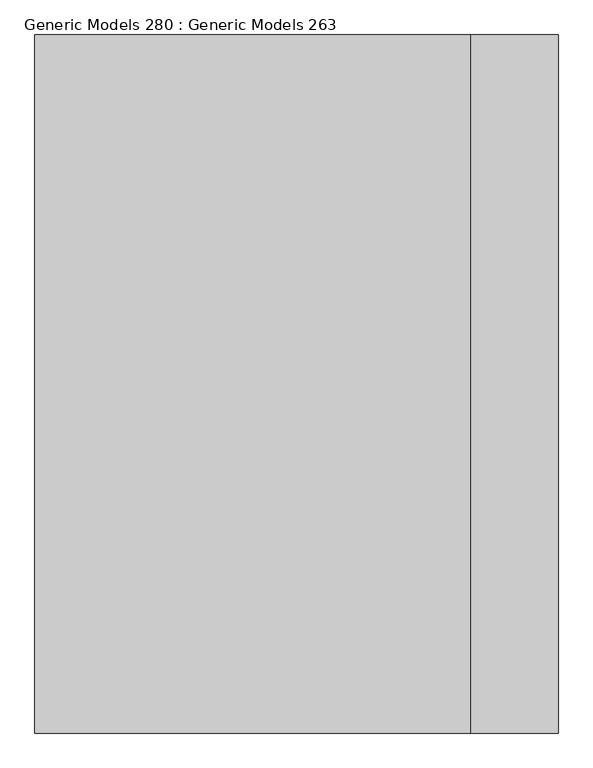
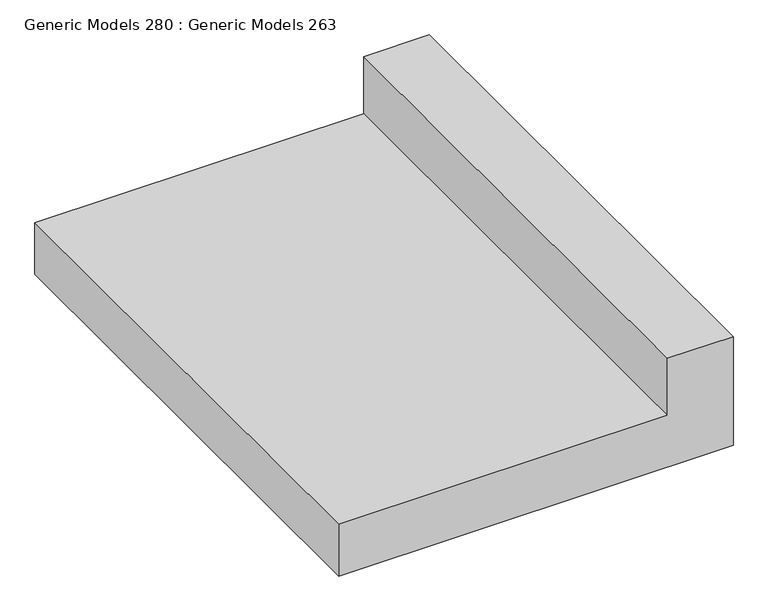
"""IFC4 building model written with IfcOpenShell, lengths in millimetres: proxy geometry, Generic Models 280 : Generic Models 263."""

import ifcopenshell
import ifcopenshell.guid

model = None  # the IFC model being written
_history = None  # IfcOwnerHistory: only IFC2X3 demands one
_inside = {}  # id of a spatial element -> (the spatial element, [elements in it])
_under = {}  # id of a project, library or spatial element -> (it, [spatial elements below it])
_declared = {}  # id of a project -> (the project, [libraries it declares])
_typed = {}  # id of a type object -> (the type object, [elements of that type])
_made_of = {}  # id of a material, layer set ... -> (it, [elements and type objects made of it])


def new_model(schema):
    """Start an empty IFC model of exactly this schema.

    Asked for "IFC4X3", IfcOpenShell would pick the latest addendum, in which some entities
    have other attributes; the version numbers below select the first issue.
    IFC2X3 requires an IfcOwnerHistory on every rooted entity: one is made here for all.
    """
    global model, _history
    if schema == "IFC4X3":
        model = ifcopenshell.file(schema_version=(4, 3, 0, 0))
    else:
        model = ifcopenshell.file(schema=schema)
    _inside.clear()
    _under.clear()
    _declared.clear()
    _typed.clear()
    _made_of.clear()
    _history = None
    if model.schema == "IFC2X3":
        org = make("IfcOrganization", Name="unknown")
        user = make(
            "IfcPersonAndOrganization",
            ThePerson=make("IfcPerson", FamilyName="unknown"),
            TheOrganization=org,
        )
        app = make(
            "IfcApplication",
            ApplicationDeveloper=org,
            Version="unknown",
            ApplicationFullName="unknown",
            ApplicationIdentifier="unknown",
        )
        _history = make(
            "IfcOwnerHistory",
            OwningUser=user,
            OwningApplication=app,
            ChangeAction="ADDED",
            CreationDate=0,
        )
    return model


def make(cls, **values):
    """One entity of the class cls with the attributes given. An attribute that is None is left unset."""
    return model.create_entity(
        cls, **{name: value for name, value in values.items() if value is not None}
    )


def rooted(cls, **values):
    """An entity with a GlobalId (a new one), such as an element, a storey or a relation."""
    return make(cls, GlobalId=ifcopenshell.guid.new(), OwnerHistory=_history, **values)


def si_unit(unit_type, name, prefix=None):
    """IfcSIUnit, for example si_unit("LENGTHUNIT", "METRE", prefix="MILLI")."""
    return make("IfcSIUnit", UnitType=unit_type, Prefix=prefix, Name=name)


def assignment(units):
    """IfcUnitAssignment: the units of a project."""
    return None if units is None else make("IfcUnitAssignment", Units=units)


def point(xyz):
    """IfcCartesianPoint."""
    return None if xyz is None else make("IfcCartesianPoint", Coordinates=xyz)


def direction(xyz):
    """IfcDirection."""
    return None if xyz is None else make("IfcDirection", DirectionRatios=xyz)


def frame(location, z_axis=None, x_axis=None):
    """IfcAxis2Placement3D, a coordinate frame: its origin and axes. An axis left out is left unset."""
    return make(
        "IfcAxis2Placement3D",
        Location=point(location),
        Axis=direction(z_axis),
        RefDirection=direction(x_axis),
    )


def origin():
    """The frame at (0, 0, 0) with its axes left unset."""
    return frame((0.0, 0.0, 0.0))


def place(relative_to, where):
    """IfcLocalPlacement: puts the frame where relative to a parent placement (None: the world)."""
    return make(
        "IfcLocalPlacement", PlacementRelTo=relative_to, RelativePlacement=where
    )


def context(
    kind, dimensions, precision=None, world=None, true_north=None, identifier=None
):
    """IfcGeometricRepresentationContext, for example the 3D "Model" context."""
    return make(
        "IfcGeometricRepresentationContext",
        ContextIdentifier=identifier,
        ContextType=kind,
        CoordinateSpaceDimension=dimensions,
        Precision=precision,
        WorldCoordinateSystem=world,
        TrueNorth=true_north,
    )


def project(units=None, contexts=None):
    """IfcProject with its units and contexts."""
    return rooted(
        "IfcProject",
        Name="project",
        RepresentationContexts=contexts,
        UnitsInContext=assignment(units),
    )


def spatial(cls, under=None, at=None, **own):
    """A site, building, storey or space (cls), placed at a placement, below another one or the project."""
    s = rooted(cls, ObjectPlacement=at, **own)
    if under is not None:
        _under.setdefault(under.id(), (under, []))[1].append(s)
    return s


def polyline(points):
    """IfcPolyline through the points."""
    return make("IfcPolyline", Points=[point(p) for p in points])


def outline(outer, holes=None, kind="AREA"):
    """IfcArbitraryClosedProfileDef: a profile drawn as a closed curve; with holes, ...WithVoids."""
    if holes is None:
        return make("IfcArbitraryClosedProfileDef", ProfileType=kind, OuterCurve=outer)
    return make(
        "IfcArbitraryProfileDefWithVoids",
        ProfileType=kind,
        OuterCurve=outer,
        InnerCurves=holes,
    )


def extrude(swept, where, along, depth):
    """IfcExtrudedAreaSolid: the profile swept, set in the frame where, extruded along a direction by depth."""
    return make(
        "IfcExtrudedAreaSolid",
        SweptArea=swept,
        Position=where,
        ExtrudedDirection=direction(along),
        Depth=depth,
    )


def shape(context_of_items, identifier, shape_type, items):
    """IfcShapeRepresentation: the items that make up one representation, for example the "Body"."""
    return make(
        "IfcShapeRepresentation",
        ContextOfItems=context_of_items,
        RepresentationIdentifier=identifier,
        RepresentationType=shape_type,
        Items=items,
    )


def source(mapping_origin, context_of_items, identifier, shape_type, items):
    """IfcRepresentationMap: a shape defined once, which mapped items show again and again."""
    return make(
        "IfcRepresentationMap",
        MappingOrigin=mapping_origin,
        MappedRepresentation=shape(context_of_items, identifier, shape_type, items),
    )


def transform(
    local_origin,
    x_axis=None,
    y_axis=None,
    z_axis=None,
    scale=None,
    scale2=None,
    scale3=None,
    uniform=True,
):
    """IfcCartesianTransformationOperator3D, or its non-uniform kind. x_axis, y_axis, z_axis: its Axis1, 2, 3."""
    if uniform:
        return make(
            "IfcCartesianTransformationOperator3D",
            Axis1=direction(x_axis),
            Axis2=direction(y_axis),
            LocalOrigin=point(local_origin),
            Scale=scale,
            Axis3=direction(z_axis),
        )
    return make(
        "IfcCartesianTransformationOperator3DnonUniform",
        Axis1=direction(x_axis),
        Axis2=direction(y_axis),
        LocalOrigin=point(local_origin),
        Scale=scale,
        Axis3=direction(z_axis),
        Scale2=scale2,
        Scale3=scale3,
    )


def mapped(mapping_source, mapping_target):
    """IfcMappedItem: shows the shape of a source again, moved by a transform."""
    return make(
        "IfcMappedItem", MappingSource=mapping_source, MappingTarget=mapping_target
    )


def made_of(thing, what):
    """Note that an element or type object is made of a material, layer set ...; save() writes the relation."""
    if what is not None:
        _made_of.setdefault(what.id(), (what, []))[1].append(thing)
    return thing


def element(
    cls,
    number,
    at=None,
    inside=None,
    cuts=None,
    type_object=None,
    material=None,
    context=None,
    identifier="Body",
    shape_type=None,
    held_by="IfcProductDefinitionShape",
    body=None,
    shapes=None,
    **own,
):
    """One element of the class cls, such as IfcWall. Its Tag is "e" and its number.

    at: its placement. inside: the storey or other place that contains it. cuts: it is an
    opening in that element (IfcRelVoidsElement). A single representation is given by context,
    identifier, shape_type and body (its items); several are given by shapes. held_by: the class
    of the entity that holds the representations. save() writes the other relations.
    """
    e = rooted(cls, Tag="e%d" % number, ObjectPlacement=at, **own)
    if body is not None:
        shapes = [shape(context, identifier, shape_type, body)]
    if shapes is not None:
        e.Representation = make(held_by, Representations=shapes)
    if inside is not None:
        _inside.setdefault(inside.id(), (inside, []))[1].append(e)
    if cuts is not None:
        rooted(
            "IfcRelVoidsElement", RelatingBuildingElement=cuts, RelatedOpeningElement=e
        )
    if type_object is not None:
        _typed.setdefault(type_object.id(), (type_object, []))[1].append(e)
    return made_of(e, material)


def aggregate(whole, parts):
    """IfcRelAggregates: a whole, such as a stair, and the parts it consists of."""
    return rooted("IfcRelAggregates", RelatingObject=whole, RelatedObjects=parts)


def save(model, path):
    """Write the relations noted so far, then the file.

    IfcRelAggregates (storeys below a building ...), IfcRelContainedInSpatialStructure (elements
    in a storey), IfcRelDefinesByType, IfcRelAssociatesMaterial and IfcRelDeclares: one each for
    every whole, place, type object, material and project.
    """
    for whole, parts in _under.values():
        aggregate(whole, parts)
    for where, things in _inside.values():
        rooted(
            "IfcRelContainedInSpatialStructure",
            RelatedElements=things,
            RelatingStructure=where,
        )
    for kind, things in _typed.values():
        rooted("IfcRelDefinesByType", RelatedObjects=things, RelatingType=kind)
    for what, things in _made_of.values():
        rooted("IfcRelAssociatesMaterial", RelatedObjects=things, RelatingMaterial=what)
    for by, libraries in _declared.values():
        rooted("IfcRelDeclares", RelatingContext=by, RelatedDefinitions=libraries)
    model.write(path)


def generic_models_280_generic_models_263_4ff5fa89(model_context):
    return source(origin(), model_context, "Body", "SweptSolid", [
        extrude(outline(polyline([(-381.0, 62776.3797726), (-381.0, 62014.3797726), (-508.0, 62014.3797726), (-508.0, 62928.7797726), (-241.3, 62928.7797726), (-241.3, 62776.3797726), (-381.0, 62776.3797726)])), frame((0.0, -94.4486541, 0.0), z_axis=(0.0, 1.0, 0.0), x_axis=(0.0, 0.0, 1.0)), (0.0, 0.0, 1.0), 1219.2),
    ])


if __name__ == "__main__":
    model = new_model("IFC4")
    model_context = context("Model", 3, world=origin())
    ifc_project = project(units=[si_unit("LENGTHUNIT", "METRE", prefix="MILLI")], contexts=[model_context])
    site = spatial("IfcSite", under=ifc_project)
    building = spatial("IfcBuilding", under=site)
    placement = place(None, origin())
    generic_models_280_generic_models_263_shape = generic_models_280_generic_models_263_4ff5fa89(model_context)
    element("IfcBuildingElementProxy", 1, Name="Generic Models 280 : Generic Models 263", ObjectType="Generic Models 280 : Generic Models 263", at=placement, inside=building, context=model_context, shape_type="MappedRepresentation", body=[
        mapped(generic_models_280_generic_models_263_shape, transform((0.0, 0.0, 0.0), x_axis=(1.0, 0.0, 0.0), y_axis=(0.0, 1.0, 0.0), z_axis=(0.0, 0.0, 1.0))),
    ])
    save(model, "model.ifc")

# Revit data of these elements
# Element 1 (IfcBuildingElementProxy, "Generic Models 280 : Generic Models 263")
#   Materials on its faces: "5\" MIN. COMPACTED BASE AGGREGATE UNDER CURB"
# Materials
#   "5\" MIN. COMPACTED BASE AGGREGATE UNDER CURB": class "Miscellaneous", colour RGB 183 184 198, transparency 0, Cost = 0
